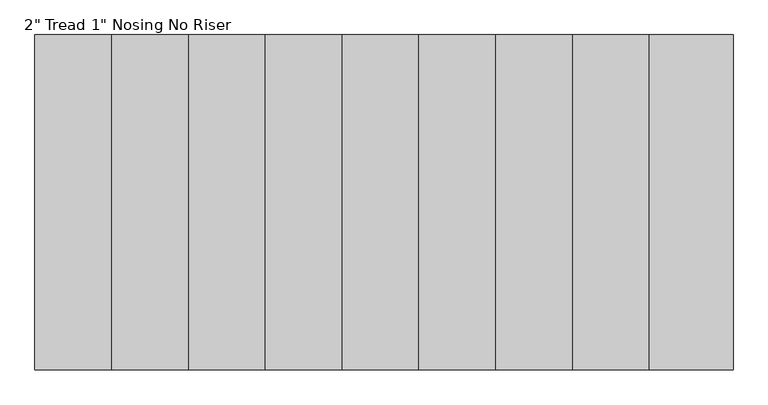
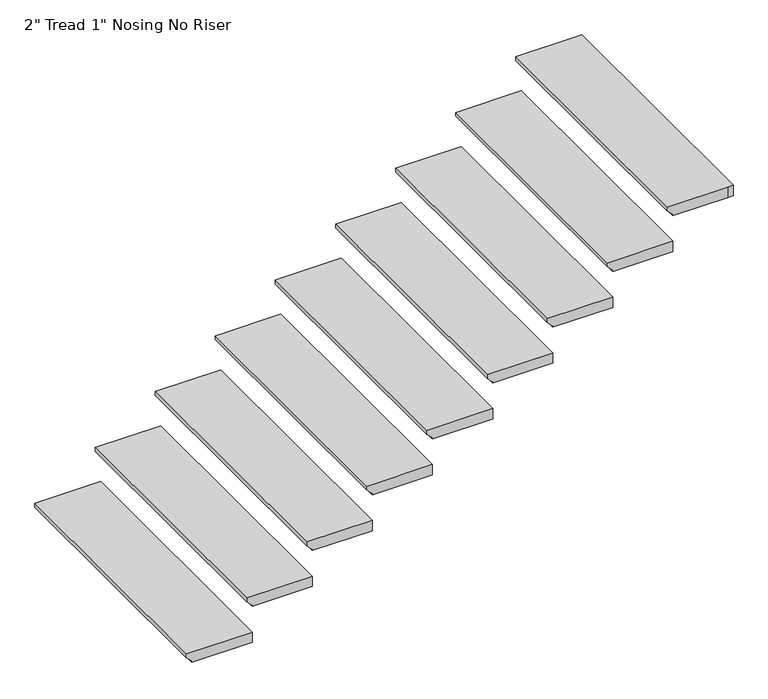
"""IFC4 building model written with IfcOpenShell, lengths in millimetres: stair flight geometry."""

import ifcopenshell
import ifcopenshell.guid

model = None  # the IFC model being written
_history = None  # IfcOwnerHistory: only IFC2X3 demands one
_inside = {}  # id of a spatial element -> (the spatial element, [elements in it])
_under = {}  # id of a project, library or spatial element -> (it, [spatial elements below it])
_declared = {}  # id of a project -> (the project, [libraries it declares])
_typed = {}  # id of a type object -> (the type object, [elements of that type])
_made_of = {}  # id of a material, layer set ... -> (it, [elements and type objects made of it])


def new_model(schema):
    """Start an empty IFC model of exactly this schema.

    Asked for "IFC4X3", IfcOpenShell would pick the latest addendum, in which some entities
    have other attributes; the version numbers below select the first issue.
    IFC2X3 requires an IfcOwnerHistory on every rooted entity: one is made here for all.
    """
    global model, _history
    if schema == "IFC4X3":
        model = ifcopenshell.file(schema_version=(4, 3, 0, 0))
    else:
        model = ifcopenshell.file(schema=schema)
    _inside.clear()
    _under.clear()
    _declared.clear()
    _typed.clear()
    _made_of.clear()
    _history = None
    if model.schema == "IFC2X3":
        org = make("IfcOrganization", Name="unknown")
        user = make(
            "IfcPersonAndOrganization",
            ThePerson=make("IfcPerson", FamilyName="unknown"),
            TheOrganization=org,
        )
        app = make(
            "IfcApplication",
            ApplicationDeveloper=org,
            Version="unknown",
            ApplicationFullName="unknown",
            ApplicationIdentifier="unknown",
        )
        _history = make(
            "IfcOwnerHistory",
            OwningUser=user,
            OwningApplication=app,
            ChangeAction="ADDED",
            CreationDate=0,
        )
    return model


def make(cls, **values):
    """One entity of the class cls with the attributes given. An attribute that is None is left unset."""
    return model.create_entity(
        cls, **{name: value for name, value in values.items() if value is not None}
    )


def rooted(cls, **values):
    """An entity with a GlobalId (a new one), such as an element, a storey or a relation."""
    return make(cls, GlobalId=ifcopenshell.guid.new(), OwnerHistory=_history, **values)


def si_unit(unit_type, name, prefix=None):
    """IfcSIUnit, for example si_unit("LENGTHUNIT", "METRE", prefix="MILLI")."""
    return make("IfcSIUnit", UnitType=unit_type, Prefix=prefix, Name=name)


def assignment(units):
    """IfcUnitAssignment: the units of a project."""
    return None if units is None else make("IfcUnitAssignment", Units=units)


def point(xyz):
    """IfcCartesianPoint."""
    return None if xyz is None else make("IfcCartesianPoint", Coordinates=xyz)


def direction(xyz):
    """IfcDirection."""
    return None if xyz is None else make("IfcDirection", DirectionRatios=xyz)


def frame(location, z_axis=None, x_axis=None):
    """IfcAxis2Placement3D, a coordinate frame: its origin and axes. An axis left out is left unset."""
    return make(
        "IfcAxis2Placement3D",
        Location=point(location),
        Axis=direction(z_axis),
        RefDirection=direction(x_axis),
    )


def origin():
    """The frame at (0, 0, 0) with its axes left unset."""
    return frame((0.0, 0.0, 0.0))


def place(relative_to, where):
    """IfcLocalPlacement: puts the frame where relative to a parent placement (None: the world)."""
    return make(
        "IfcLocalPlacement", PlacementRelTo=relative_to, RelativePlacement=where
    )


def context(
    kind, dimensions, precision=None, world=None, true_north=None, identifier=None
):
    """IfcGeometricRepresentationContext, for example the 3D "Model" context."""
    return make(
        "IfcGeometricRepresentationContext",
        ContextIdentifier=identifier,
        ContextType=kind,
        CoordinateSpaceDimension=dimensions,
        Precision=precision,
        WorldCoordinateSystem=world,
        TrueNorth=true_north,
    )


def project(units=None, contexts=None):
    """IfcProject with its units and contexts."""
    return rooted(
        "IfcProject",
        Name="project",
        RepresentationContexts=contexts,
        UnitsInContext=assignment(units),
    )


def spatial(cls, under=None, at=None, **own):
    """A site, building, storey or space (cls), placed at a placement, below another one or the project."""
    s = rooted(cls, ObjectPlacement=at, **own)
    if under is not None:
        _under.setdefault(under.id(), (under, []))[1].append(s)
    return s


def faces_of(points, faces, orient=None, outer=None):
    """IfcFace entities. A face is a list of loops; a loop is a list of indices into points, from 0.

    orient and outer hold one flag for each loop. By default every Orientation is true, the
    first loop of a face is its IfcFaceOuterBound and the others are IfcFaceBound.
    """
    made = []
    for i, loops in enumerate(faces):
        bounds = []
        for j, loop in enumerate(loops):
            is_outer = j == 0 if outer is None else outer[i][j]
            bounds.append(
                make(
                    "IfcFaceOuterBound" if is_outer else "IfcFaceBound",
                    Bound=make("IfcPolyLoop", Polygon=[points[k] for k in loop]),
                    Orientation=True if orient is None else orient[i][j],
                )
            )
        made.append(make("IfcFace", Bounds=bounds))
    return made


def faceted_brep(points, faces, orient=None, outer=None, voids=None):
    """IfcFacetedBrep: a solid bounded by flat faces; with voids (closed shells), ...WithVoids."""
    shared = [point(p) for p in points]
    hull = make("IfcClosedShell", CfsFaces=faces_of(shared, faces, orient, outer))
    if voids is None:
        return make("IfcFacetedBrep", Outer=hull)
    return make(
        "IfcFacetedBrepWithVoids",
        Outer=hull,
        Voids=[
            make(cls, CfsFaces=faces_of(shared, fs, o, b)) for cls, fs, o, b in voids
        ],
    )


def shape(context_of_items, identifier, shape_type, items):
    """IfcShapeRepresentation: the items that make up one representation, for example the "Body"."""
    return make(
        "IfcShapeRepresentation",
        ContextOfItems=context_of_items,
        RepresentationIdentifier=identifier,
        RepresentationType=shape_type,
        Items=items,
    )


def source(mapping_origin, context_of_items, identifier, shape_type, items):
    """IfcRepresentationMap: a shape defined once, which mapped items show again and again."""
    return make(
        "IfcRepresentationMap",
        MappingOrigin=mapping_origin,
        MappedRepresentation=shape(context_of_items, identifier, shape_type, items),
    )


def transform(
    local_origin,
    x_axis=None,
    y_axis=None,
    z_axis=None,
    scale=None,
    scale2=None,
    scale3=None,
    uniform=True,
):
    """IfcCartesianTransformationOperator3D, or its non-uniform kind. x_axis, y_axis, z_axis: its Axis1, 2, 3."""
    if uniform:
        return make(
            "IfcCartesianTransformationOperator3D",
            Axis1=direction(x_axis),
            Axis2=direction(y_axis),
            LocalOrigin=point(local_origin),
            Scale=scale,
            Axis3=direction(z_axis),
        )
    return make(
        "IfcCartesianTransformationOperator3DnonUniform",
        Axis1=direction(x_axis),
        Axis2=direction(y_axis),
        LocalOrigin=point(local_origin),
        Scale=scale,
        Axis3=direction(z_axis),
        Scale2=scale2,
        Scale3=scale3,
    )


def mapped(mapping_source, mapping_target):
    """IfcMappedItem: shows the shape of a source again, moved by a transform."""
    return make(
        "IfcMappedItem", MappingSource=mapping_source, MappingTarget=mapping_target
    )


def made_of(thing, what):
    """Note that an element or type object is made of a material, layer set ...; save() writes the relation."""
    if what is not None:
        _made_of.setdefault(what.id(), (what, []))[1].append(thing)
    return thing


def element(
    cls,
    number,
    at=None,
    inside=None,
    cuts=None,
    type_object=None,
    material=None,
    context=None,
    identifier="Body",
    shape_type=None,
    held_by="IfcProductDefinitionShape",
    body=None,
    shapes=None,
    **own,
):
    """One element of the class cls, such as IfcWall. Its Tag is "e" and its number.

    at: its placement. inside: the storey or other place that contains it. cuts: it is an
    opening in that element (IfcRelVoidsElement). A single representation is given by context,
    identifier, shape_type and body (its items); several are given by shapes. held_by: the class
    of the entity that holds the representations. save() writes the other relations.
    """
    e = rooted(cls, Tag="e%d" % number, ObjectPlacement=at, **own)
    if body is not None:
        shapes = [shape(context, identifier, shape_type, body)]
    if shapes is not None:
        e.Representation = make(held_by, Representations=shapes)
    if inside is not None:
        _inside.setdefault(inside.id(), (inside, []))[1].append(e)
    if cuts is not None:
        rooted(
            "IfcRelVoidsElement", RelatingBuildingElement=cuts, RelatedOpeningElement=e
        )
    if type_object is not None:
        _typed.setdefault(type_object.id(), (type_object, []))[1].append(e)
    return made_of(e, material)


def aggregate(whole, parts):
    """IfcRelAggregates: a whole, such as a stair, and the parts it consists of."""
    return rooted("IfcRelAggregates", RelatingObject=whole, RelatedObjects=parts)


def save(model, path):
    """Write the relations noted so far, then the file.

    IfcRelAggregates (storeys below a building ...), IfcRelContainedInSpatialStructure (elements
    in a storey), IfcRelDefinesByType, IfcRelAssociatesMaterial and IfcRelDeclares: one each for
    every whole, place, type object, material and project.
    """
    for whole, parts in _under.values():
        aggregate(whole, parts)
    for where, things in _inside.values():
        rooted(
            "IfcRelContainedInSpatialStructure",
            RelatedElements=things,
            RelatingStructure=where,
        )
    for kind, things in _typed.values():
        rooted("IfcRelDefinesByType", RelatedObjects=things, RelatingType=kind)
    for what, things in _made_of.values():
        rooted("IfcRelAssociatesMaterial", RelatedObjects=things, RelatingMaterial=what)
    for by, libraries in _declared.values():
        rooted("IfcRelDeclares", RelatingContext=by, RelatedDefinitions=libraries)
    model.write(path)


def stair_flight_2cb6126d(model_context):
    return source(origin(), model_context, "Body", "Brep", [
        faceted_brep([(17790.1956761, -8619.1304995, 30637.6456522), (17790.1956761, -8619.1304995, 30656.6956522), (17790.1956761, -7399.9304995, 30656.6956522), (17790.1956761, -7399.9304995, 30637.6456522), (17815.5956761, -8619.1304995, 30612.2456522), (17815.5956761, -7399.9304995, 30612.2456522), (18094.9956761, -8619.1304995, 30656.6956522), (18094.9956761, -7399.9304995, 30656.6956522), (17815.5956761, -7399.9304995, 30605.8956522), (18094.9956761, -7399.9304995, 30605.8956522), (18094.9956761, -8619.1304995, 30605.8956522), (17815.5956761, -8619.1304995, 30605.8956522)], [[[0, 1, 2, 3]], [[4, 0, 3, 5]], [[2, 1, 6, 7]], [[8, 9, 10, 11]], [[2, 7, 9, 8, 5, 3]], [[8, 11, 4, 5]], [[6, 1, 0, 4, 11, 10]], [[7, 6, 10, 9]]]),
        faceted_brep([(18069.5956761, -7399.9304995, 30833.3913043), (18069.5956761, -8619.1304995, 30833.3913043), (18374.3956761, -8619.1304995, 30833.3913043), (18374.3956761, -7399.9304995, 30833.3913043), (18094.9956761, -7399.9304995, 30782.5913043), (18374.3956761, -7399.9304995, 30782.5913043), (18374.3956761, -8619.1304995, 30782.5913043), (18094.9956761, -8619.1304995, 30782.5913043), (18094.9956761, -7399.9304995, 30788.9413043), (18069.5956761, -7399.9304995, 30814.3413043), (18094.9956761, -8619.1304995, 30788.9413043), (18069.5956761, -8619.1304995, 30814.3413043)], [[[0, 1, 2, 3]], [[4, 5, 6, 7]], [[0, 3, 5, 4, 8, 9]], [[4, 7, 10, 8]], [[2, 1, 11, 10, 7, 6]], [[3, 2, 6, 5]], [[11, 1, 0, 9]], [[10, 11, 9, 8]]]),
        faceted_brep([(18348.9956761, -7399.9304995, 31010.0869565), (18348.9956761, -8619.1304995, 31010.0869565), (18653.7956761, -8619.1304995, 31010.0869565), (18653.7956761, -7399.9304995, 31010.0869565), (18374.3956761, -7399.9304995, 30959.2869565), (18653.7956761, -7399.9304995, 30959.2869565), (18653.7956761, -8619.1304995, 30959.2869565), (18374.3956761, -8619.1304995, 30959.2869565), (18374.3956761, -7399.9304995, 30965.6369565), (18348.9956761, -7399.9304995, 30991.0369565), (18374.3956761, -8619.1304995, 30965.6369565), (18348.9956761, -8619.1304995, 30991.0369565)], [[[0, 1, 2, 3]], [[4, 5, 6, 7]], [[0, 3, 5, 4, 8, 9]], [[4, 7, 10, 8]], [[2, 1, 11, 10, 7, 6]], [[3, 2, 6, 5]], [[11, 1, 0, 9]], [[10, 11, 9, 8]]]),
        faceted_brep([(18628.3956761, -7399.9304995, 31186.7826087), (18628.3956761, -8619.1304995, 31186.7826087), (18933.1956761, -8619.1304995, 31186.7826087), (18933.1956761, -7399.9304995, 31186.7826087), (18653.7956761, -7399.9304995, 31135.9826087), (18933.1956761, -7399.9304995, 31135.9826087), (18933.1956761, -8619.1304995, 31135.9826087), (18653.7956761, -8619.1304995, 31135.9826087), (18653.7956761, -7399.9304995, 31142.3326087), (18628.3956761, -7399.9304995, 31167.7326087), (18653.7956761, -8619.1304995, 31142.3326087), (18628.3956761, -8619.1304995, 31167.7326087)], [[[0, 1, 2, 3]], [[4, 5, 6, 7]], [[0, 3, 5, 4, 8, 9]], [[4, 7, 10, 8]], [[2, 1, 11, 10, 7, 6]], [[3, 2, 6, 5]], [[11, 1, 0, 9]], [[10, 11, 9, 8]]]),
        faceted_brep([(18907.7956761, -7399.9304995, 31363.4782609), (18907.7956761, -8619.1304995, 31363.4782609), (19212.5956761, -8619.1304995, 31363.4782609), (19212.5956761, -7399.9304995, 31363.4782609), (18933.1956761, -7399.9304995, 31312.6782609), (19212.5956761, -7399.9304995, 31312.6782609), (19212.5956761, -8619.1304995, 31312.6782609), (18933.1956761, -8619.1304995, 31312.6782609), (18933.1956761, -7399.9304995, 31319.0282609), (18907.7956761, -7399.9304995, 31344.4282609), (18933.1956761, -8619.1304995, 31319.0282609), (18907.7956761, -8619.1304995, 31344.4282609)], [[[0, 1, 2, 3]], [[4, 5, 6, 7]], [[0, 3, 5, 4, 8, 9]], [[4, 7, 10, 8]], [[2, 1, 11, 10, 7, 6]], [[3, 2, 6, 5]], [[11, 1, 0, 9]], [[10, 11, 9, 8]]]),
        faceted_brep([(19187.1956761, -7399.9304995, 31540.173913), (19187.1956761, -8619.1304995, 31540.173913), (19491.9956761, -8619.1304995, 31540.173913), (19491.9956761, -7399.9304995, 31540.173913), (19212.5956761, -7399.9304995, 31489.373913), (19491.9956761, -7399.9304995, 31489.373913), (19491.9956761, -8619.1304995, 31489.373913), (19212.5956761, -8619.1304995, 31489.373913), (19212.5956761, -7399.9304995, 31495.723913), (19187.1956761, -7399.9304995, 31521.123913), (19212.5956761, -8619.1304995, 31495.723913), (19187.1956761, -8619.1304995, 31521.123913)], [[[0, 1, 2, 3]], [[4, 5, 6, 7]], [[0, 3, 5, 4, 8, 9]], [[4, 7, 10, 8]], [[2, 1, 11, 10, 7, 6]], [[3, 2, 6, 5]], [[11, 1, 0, 9]], [[10, 11, 9, 8]]]),
        faceted_brep([(19466.5956761, -7399.9304995, 31716.8695652), (19466.5956761, -8619.1304995, 31716.8695652), (19771.3956761, -8619.1304995, 31716.8695652), (19771.3956761, -7399.9304995, 31716.8695652), (19491.9956761, -7399.9304995, 31666.0695652), (19771.3956761, -7399.9304995, 31666.0695652), (19771.3956761, -8619.1304995, 31666.0695652), (19491.9956761, -8619.1304995, 31666.0695652), (19491.9956761, -7399.9304995, 31672.4195652), (19466.5956761, -7399.9304995, 31697.8195652), (19491.9956761, -8619.1304995, 31672.4195652), (19466.5956761, -8619.1304995, 31697.8195652)], [[[0, 1, 2, 3]], [[4, 5, 6, 7]], [[0, 3, 5, 4, 8, 9]], [[4, 7, 10, 8]], [[2, 1, 11, 10, 7, 6]], [[3, 2, 6, 5]], [[11, 1, 0, 9]], [[10, 11, 9, 8]]]),
        faceted_brep([(19745.9956761, -7399.9304995, 31893.5652174), (19745.9956761, -8619.1304995, 31893.5652174), (20050.7956761, -8619.1304995, 31893.5652174), (20050.7956761, -7399.9304995, 31893.5652174), (19771.3956761, -7399.9304995, 31842.7652174), (20050.7956761, -7399.9304995, 31842.7652174), (20050.7956761, -8619.1304995, 31842.7652174), (19771.3956761, -8619.1304995, 31842.7652174), (19771.3956761, -7399.9304995, 31849.1152174), (19745.9956761, -7399.9304995, 31874.5152174), (19771.3956761, -8619.1304995, 31849.1152174), (19745.9956761, -8619.1304995, 31874.5152174)], [[[0, 1, 2, 3]], [[4, 5, 6, 7]], [[0, 3, 5, 4, 8, 9]], [[4, 7, 10, 8]], [[2, 1, 11, 10, 7, 6]], [[3, 2, 6, 5]], [[11, 1, 0, 9]], [[10, 11, 9, 8]]]),
        faceted_brep([(20330.1956761, -7399.9304995, 32070.2608696), (20304.7956761, -7399.9304995, 32070.2608696), (20025.3956761, -7399.9304995, 32070.2608696), (20025.3956761, -8619.1304995, 32070.2608696), (20304.7956761, -8619.1304995, 32070.2608696), (20330.1956761, -8619.1304995, 32070.2608696), (20304.7956761, -7399.9304995, 32019.4608696), (20330.1956761, -7399.9304995, 32019.4608696), (20330.1956761, -8619.1304995, 32019.4608696), (20304.7956761, -8619.1304995, 32019.4608696), (20050.7956761, -8619.1304995, 32019.4608696), (20050.7956761, -7399.9304995, 32019.4608696), (20050.7956761, -7399.9304995, 32025.8108696), (20025.3956761, -7399.9304995, 32051.2108696), (20050.7956761, -8619.1304995, 32025.8108696), (20025.3956761, -8619.1304995, 32051.2108696)], [[[0, 1, 2, 3, 4, 5]], [[6, 7, 8, 9, 10, 11]], [[1, 0, 7, 6]], [[2, 1, 6, 11, 12, 13]], [[11, 10, 14, 12]], [[4, 3, 15, 14, 10, 9]], [[5, 4, 9, 8]], [[0, 5, 8, 7]], [[15, 3, 2, 13]], [[14, 15, 13, 12]]]),
    ])


if __name__ == "__main__":
    model = new_model("IFC4")
    model_context = context("Model", 3, world=origin())
    ifc_project = project(units=[si_unit("LENGTHUNIT", "METRE", prefix="MILLI")], contexts=[model_context])
    site = spatial("IfcSite", under=ifc_project)
    building = spatial("IfcBuilding", under=site)
    placement = place(None, origin())
    stair_flight_shape = stair_flight_2cb6126d(model_context)
    element("IfcStairFlight", 1, ObjectType="2\" Tread 1\" Nosing No Riser", at=placement, inside=building, context=model_context, shape_type="MappedRepresentation", body=[
        mapped(stair_flight_shape, transform((0.0, 0.0, 0.0), x_axis=(1.0, 0.0, 0.0), y_axis=(0.0, 1.0, 0.0), z_axis=(0.0, 0.0, 1.0))),
    ])
    save(model, "model.ifc")

# Revit data of these elements
# Project information
#   Organization Name = "Gannett Fleming, Inc."
#   Building Name = "Health Center"
#   Project Issue Date = "April 1, 2021"
#   Project Status = "04-01-21 ARCHITECTURAL CHECK SET"
#   Client Name = "Autodesk"
#   Project Address = "Enter address here"
#   Project Name = "Revit 2021\nDataset Model"
#   Project Number = "056750"
